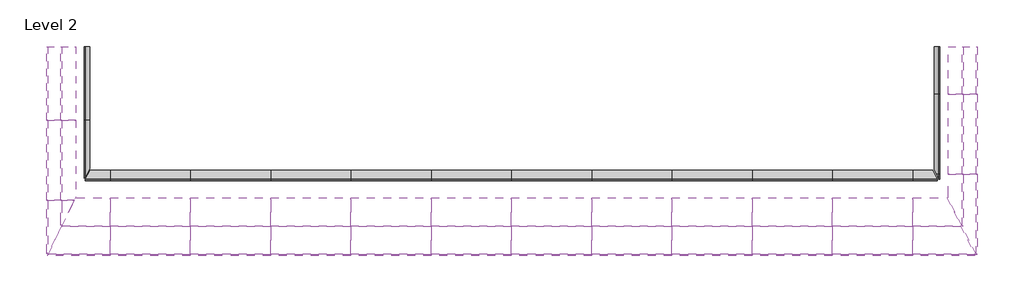
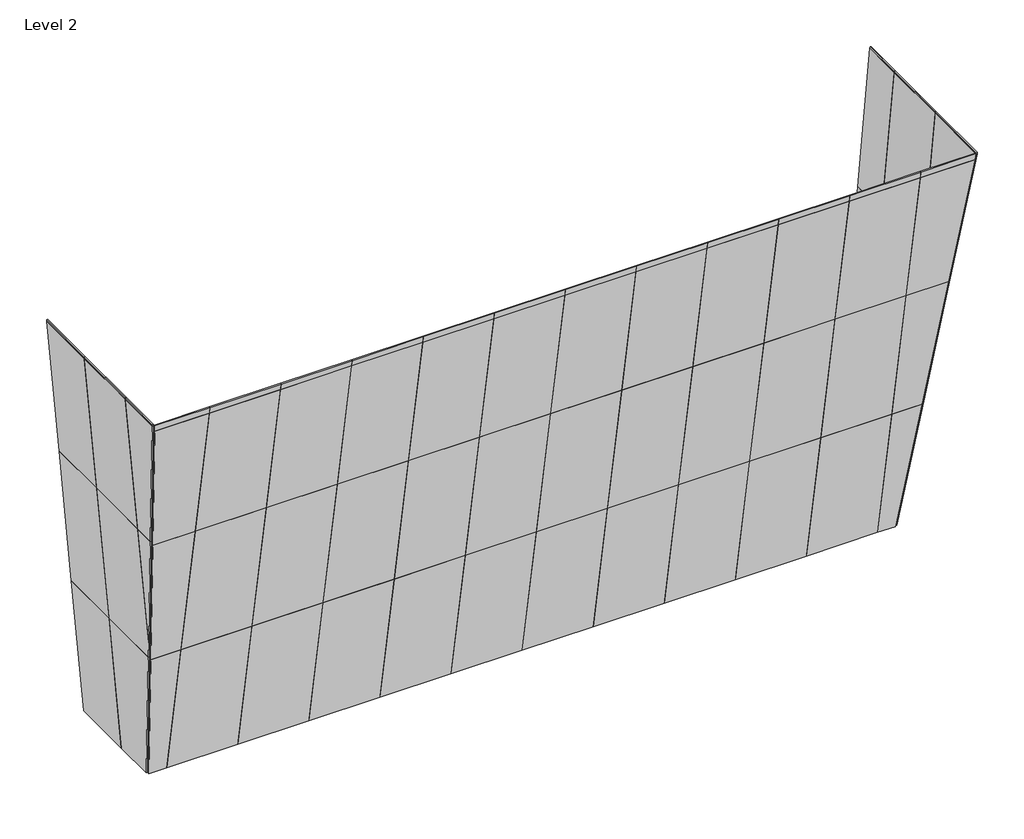
# One storey: 71 plates.
"""IFC4 building model written with IfcOpenShell, lengths in millimetres."""

import ifcopenshell
import ifcopenshell.guid

model = None  # the IFC model being written
_history = None  # IfcOwnerHistory: only IFC2X3 demands one
_inside = {}  # id of a spatial element -> (the spatial element, [elements in it])
_under = {}  # id of a project, library or spatial element -> (it, [spatial elements below it])
_declared = {}  # id of a project -> (the project, [libraries it declares])
_typed = {}  # id of a type object -> (the type object, [elements of that type])
_made_of = {}  # id of a material, layer set ... -> (it, [elements and type objects made of it])


def new_model(schema):
    """Start an empty IFC model of exactly this schema.

    Asked for "IFC4X3", IfcOpenShell would pick the latest addendum, in which some entities
    have other attributes; the version numbers below select the first issue.
    IFC2X3 requires an IfcOwnerHistory on every rooted entity: one is made here for all.
    """
    global model, _history
    if schema == "IFC4X3":
        model = ifcopenshell.file(schema_version=(4, 3, 0, 0))
    else:
        model = ifcopenshell.file(schema=schema)
    _inside.clear()
    _under.clear()
    _declared.clear()
    _typed.clear()
    _made_of.clear()
    _history = None
    if model.schema == "IFC2X3":
        org = make("IfcOrganization", Name="unknown")
        user = make(
            "IfcPersonAndOrganization",
            ThePerson=make("IfcPerson", FamilyName="unknown"),
            TheOrganization=org,
        )
        app = make(
            "IfcApplication",
            ApplicationDeveloper=org,
            Version="unknown",
            ApplicationFullName="unknown",
            ApplicationIdentifier="unknown",
        )
        _history = make(
            "IfcOwnerHistory",
            OwningUser=user,
            OwningApplication=app,
            ChangeAction="ADDED",
            CreationDate=0,
        )
    return model


def make(cls, **values):
    """One entity of the class cls with the attributes given. An attribute that is None is left unset."""
    return model.create_entity(
        cls, **{name: value for name, value in values.items() if value is not None}
    )


def rooted(cls, **values):
    """An entity with a GlobalId (a new one), such as an element, a storey or a relation."""
    return make(cls, GlobalId=ifcopenshell.guid.new(), OwnerHistory=_history, **values)


def si_unit(unit_type, name, prefix=None):
    """IfcSIUnit, for example si_unit("LENGTHUNIT", "METRE", prefix="MILLI")."""
    return make("IfcSIUnit", UnitType=unit_type, Prefix=prefix, Name=name)


def assignment(units):
    """IfcUnitAssignment: the units of a project."""
    return None if units is None else make("IfcUnitAssignment", Units=units)


def point(xyz):
    """IfcCartesianPoint."""
    return None if xyz is None else make("IfcCartesianPoint", Coordinates=xyz)


def direction(xyz):
    """IfcDirection."""
    return None if xyz is None else make("IfcDirection", DirectionRatios=xyz)


def frame(location, z_axis=None, x_axis=None):
    """IfcAxis2Placement3D, a coordinate frame: its origin and axes. An axis left out is left unset."""
    return make(
        "IfcAxis2Placement3D",
        Location=point(location),
        Axis=direction(z_axis),
        RefDirection=direction(x_axis),
    )


def origin():
    """The frame at (0, 0, 0) with its axes left unset."""
    return frame((0.0, 0.0, 0.0))


def origin_with_axes():
    """The frame at (0, 0, 0) with the z axis (0, 0, 1) and the x axis (1, 0, 0) written out."""
    return frame((0.0, 0.0, 0.0), z_axis=(0.0, 0.0, 1.0), x_axis=(1.0, 0.0, 0.0))


def place(relative_to, where):
    """IfcLocalPlacement: puts the frame where relative to a parent placement (None: the world)."""
    return make(
        "IfcLocalPlacement", PlacementRelTo=relative_to, RelativePlacement=where
    )


def context(
    kind, dimensions, precision=None, world=None, true_north=None, identifier=None
):
    """IfcGeometricRepresentationContext, for example the 3D "Model" context."""
    return make(
        "IfcGeometricRepresentationContext",
        ContextIdentifier=identifier,
        ContextType=kind,
        CoordinateSpaceDimension=dimensions,
        Precision=precision,
        WorldCoordinateSystem=world,
        TrueNorth=true_north,
    )


def project(units=None, contexts=None):
    """IfcProject with its units and contexts."""
    return rooted(
        "IfcProject",
        Name="project",
        RepresentationContexts=contexts,
        UnitsInContext=assignment(units),
    )


def spatial(cls, under=None, at=None, **own):
    """A site, building, storey or space (cls), placed at a placement, below another one or the project."""
    s = rooted(cls, ObjectPlacement=at, **own)
    if under is not None:
        _under.setdefault(under.id(), (under, []))[1].append(s)
    return s


def polyline(points):
    """IfcPolyline through the points."""
    return make("IfcPolyline", Points=[point(p) for p in points])


def outline(outer, holes=None, kind="AREA"):
    """IfcArbitraryClosedProfileDef: a profile drawn as a closed curve; with holes, ...WithVoids."""
    if holes is None:
        return make("IfcArbitraryClosedProfileDef", ProfileType=kind, OuterCurve=outer)
    return make(
        "IfcArbitraryProfileDefWithVoids",
        ProfileType=kind,
        OuterCurve=outer,
        InnerCurves=holes,
    )


def extrude(swept, where, along, depth):
    """IfcExtrudedAreaSolid: the profile swept, set in the frame where, extruded along a direction by depth."""
    return make(
        "IfcExtrudedAreaSolid",
        SweptArea=swept,
        Position=where,
        ExtrudedDirection=direction(along),
        Depth=depth,
    )


def shape(context_of_items, identifier, shape_type, items):
    """IfcShapeRepresentation: the items that make up one representation, for example the "Body"."""
    return make(
        "IfcShapeRepresentation",
        ContextOfItems=context_of_items,
        RepresentationIdentifier=identifier,
        RepresentationType=shape_type,
        Items=items,
    )


def source(mapping_origin, context_of_items, identifier, shape_type, items):
    """IfcRepresentationMap: a shape defined once, which mapped items show again and again."""
    return make(
        "IfcRepresentationMap",
        MappingOrigin=mapping_origin,
        MappedRepresentation=shape(context_of_items, identifier, shape_type, items),
    )


def transform(
    local_origin,
    x_axis=None,
    y_axis=None,
    z_axis=None,
    scale=None,
    scale2=None,
    scale3=None,
    uniform=True,
):
    """IfcCartesianTransformationOperator3D, or its non-uniform kind. x_axis, y_axis, z_axis: its Axis1, 2, 3."""
    if uniform:
        return make(
            "IfcCartesianTransformationOperator3D",
            Axis1=direction(x_axis),
            Axis2=direction(y_axis),
            LocalOrigin=point(local_origin),
            Scale=scale,
            Axis3=direction(z_axis),
        )
    return make(
        "IfcCartesianTransformationOperator3DnonUniform",
        Axis1=direction(x_axis),
        Axis2=direction(y_axis),
        LocalOrigin=point(local_origin),
        Scale=scale,
        Axis3=direction(z_axis),
        Scale2=scale2,
        Scale3=scale3,
    )


def mapped(mapping_source, mapping_target):
    """IfcMappedItem: shows the shape of a source again, moved by a transform."""
    return make(
        "IfcMappedItem", MappingSource=mapping_source, MappingTarget=mapping_target
    )


def made_of(thing, what):
    """Note that an element or type object is made of a material, layer set ...; save() writes the relation."""
    if what is not None:
        _made_of.setdefault(what.id(), (what, []))[1].append(thing)
    return thing


def element(
    cls,
    number,
    at=None,
    inside=None,
    cuts=None,
    type_object=None,
    material=None,
    context=None,
    identifier="Body",
    shape_type=None,
    held_by="IfcProductDefinitionShape",
    body=None,
    shapes=None,
    **own,
):
    """One element of the class cls, such as IfcWall. Its Tag is "e" and its number.

    at: its placement. inside: the storey or other place that contains it. cuts: it is an
    opening in that element (IfcRelVoidsElement). A single representation is given by context,
    identifier, shape_type and body (its items); several are given by shapes. held_by: the class
    of the entity that holds the representations. save() writes the other relations.
    """
    e = rooted(cls, Tag="e%d" % number, ObjectPlacement=at, **own)
    if body is not None:
        shapes = [shape(context, identifier, shape_type, body)]
    if shapes is not None:
        e.Representation = make(held_by, Representations=shapes)
    if inside is not None:
        _inside.setdefault(inside.id(), (inside, []))[1].append(e)
    if cuts is not None:
        rooted(
            "IfcRelVoidsElement", RelatingBuildingElement=cuts, RelatedOpeningElement=e
        )
    if type_object is not None:
        _typed.setdefault(type_object.id(), (type_object, []))[1].append(e)
    return made_of(e, material)


def aggregate(whole, parts):
    """IfcRelAggregates: a whole, such as a stair, and the parts it consists of."""
    return rooted("IfcRelAggregates", RelatingObject=whole, RelatedObjects=parts)


def save(model, path):
    """Write the relations noted so far, then the file.

    IfcRelAggregates (storeys below a building ...), IfcRelContainedInSpatialStructure (elements
    in a storey), IfcRelDefinesByType, IfcRelAssociatesMaterial and IfcRelDeclares: one each for
    every whole, place, type object, material and project.
    """
    for whole, parts in _under.values():
        aggregate(whole, parts)
    for where, things in _inside.values():
        rooted(
            "IfcRelContainedInSpatialStructure",
            RelatedElements=things,
            RelatingStructure=where,
        )
    for kind, things in _typed.values():
        rooted("IfcRelDefinesByType", RelatedObjects=things, RelatingType=kind)
    for what, things in _made_of.values():
        rooted("IfcRelAssociatesMaterial", RelatedObjects=things, RelatingMaterial=what)
    for by, libraries in _declared.values():
        rooted("IfcRelDeclares", RelatingContext=by, RelatedDefinitions=libraries)
    model.write(path)


def system_panel_glazed_2e91cb65(model_context):
    return source(origin(), model_context, "Body", "SweptSolid", [
        extrude(outline(polyline([(838.2000002, -44.45), (-838.2000002, -44.45), (-838.2000002, -19.05), (838.2000002, -19.05), (838.2000002, -44.45)])), origin_with_axes(), (0.0, 0.0, 1.0), 3657.6),
    ])


def system_panel_glazed_41c8569a(model_context):
    return source(origin(), model_context, "Body", "SweptSolid", [
        extrude(outline(polyline([(3054.1438606, -268.2393521), (0.0, 268.2393521), (3054.1438606, 268.2393521), (3054.1438606, -268.2393521)])), frame((0.0, -44.45, 0.0), z_axis=(0.0, 1.0, 0.0), x_axis=(0.0, 0.0, 1.0)), (0.0, 0.0, 1.0), 25.4),
    ])


def system_panel_glazed_1f34555f(model_context):
    return source(origin(), model_context, "Body", "SweptSolid", [
        extrude(outline(polyline([(914.4, -44.45), (-914.4, -44.45), (-914.4, -19.05), (914.4, -19.05), (914.4, -44.45)])), origin_with_axes(), (0.0, 0.0, 1.0), 3657.6),
    ])


def system_panel_glazed_8b4ddac8(model_context):
    return source(origin(), model_context, "Body", "SweptSolid", [
        extrude(outline(polyline([(838.2000002, -44.45), (-838.2000002, -44.45), (-838.2000002, -19.05), (838.2000002, -19.05), (838.2000002, -44.45)])), origin_with_axes(), (0.0, 0.0, 1.0), 41.9143134),
    ])


def system_panel_glazed_7f82afe2(model_context):
    return source(origin(), model_context, "Body", "SweptSolid", [
        extrude(outline(polyline([(914.4, -44.45), (-914.4, -44.45), (-914.4, -19.05), (914.4, -19.05), (914.4, -44.45)])), origin_with_axes(), (0.0, 0.0, 1.0), 41.9143134),
    ])


def system_panel_glazed_f4345ae3(model_context):
    return source(origin(), model_context, "Body", "SweptSolid", [
        extrude(outline(polyline([(914.4, -44.45), (-914.4, -44.45), (-914.4, -19.05), (914.4, -19.05), (914.4, -44.45)])), origin_with_axes(), (0.0, 0.0, 1.0), 169.2731269),
    ])


def system_panel_glazed_866ab655(model_context):
    return source(origin(), model_context, "Body", "SweptSolid", [
        extrude(outline(polyline([(0.0, -808.3993064), (0.0, 914.4), (3657.6, 914.4), (3657.6, -914.4), (603.4561394, -914.4), (0.0, -808.3993064)])), frame((0.0, -44.45, 0.0), z_axis=(0.0, 1.0, 0.0), x_axis=(0.0, 0.0, 1.0)), (0.0, 0.0, 1.0), 25.4),
    ])


def system_panel_glazed_bcd6892e(model_context):
    return source(origin(), model_context, "Body", "SweptSolid", [
        extrude(outline(polyline([(0.0, 53.0003468), (0.0, 589.4790509), (3657.6, 589.4790509), (3657.6, -589.4790509), (0.0, 53.0003468)])), frame((0.0, -44.45, 0.0), z_axis=(0.0, 1.0, 0.0), x_axis=(0.0, 0.0, 1.0)), (0.0, 0.0, 1.0), 25.4),
    ])


def system_panel_glazed_e7bd2299(model_context):
    return source(origin(), model_context, "Body", "SweptSolid", [
        extrude(outline(polyline([(0.0, -268.2393521), (0.0, 910.7187498), (3657.6, 910.7187498), (3657.6, -910.7187498), (0.0, -268.2393521)])), frame((0.0, -44.45, 0.0), z_axis=(0.0, 1.0, 0.0), x_axis=(0.0, 0.0, 1.0)), (0.0, 0.0, 1.0), 25.4),
    ])


def system_panel_glazed_0a43eb3e(model_context):
    return source(origin(), model_context, "Body", "SweptSolid", [
        extrude(outline(polyline([(0.0, -907.0374994), (0.0, 914.4000002), (41.9143134, 914.4000002), (41.9143134, -914.4000002), (0.0, -907.0374994)])), frame((0.0, -44.45, 0.0), z_axis=(0.0, 1.0, 0.0), x_axis=(0.0, 0.0, 1.0)), (0.0, 0.0, 1.0), 25.4),
    ])


def system_panel_glazed_35afb83b(model_context):
    return source(origin(), model_context, "Body", "SweptSolid", [
        extrude(outline(polyline([(0.0, -71.0314805), (0.0, 386.1685195), (3657.6, 386.1685195), (3657.6, -386.1685195), (0.0, -71.0314805)])), frame((0.0, -44.45, 0.0), z_axis=(0.0, 1.0, 0.0), x_axis=(0.0, 0.0, 1.0)), (0.0, 0.0, 1.0), 25.4),
    ])


def system_panel_glazed_ca25d662(model_context):
    return source(origin(), model_context, "Body", "SweptSolid", [
        extrude(outline(polyline([(0.0, -386.1685195), (0.0, 71.0314805), (3657.6, 386.1685195), (3657.6, -386.1685195), (0.0, -386.1685195)])), frame((0.0, -44.45, 0.0), z_axis=(0.0, 1.0, 0.0), x_axis=(0.0, 0.0, 1.0)), (0.0, 0.0, 1.0), 25.4),
    ])


def system_panel_glazed_d5b9b34d(model_context):
    return source(origin(), model_context, "Body", "SweptSolid", [
        extrude(outline(polyline([(0.0, -228.6), (0.0, 543.7370389), (3657.6, 543.7370389), (3657.6, -543.7370389), (0.0, -228.6)])), frame((0.0, -44.45, 0.0), z_axis=(0.0, 1.0, 0.0), x_axis=(0.0, 0.0, 1.0)), (0.0, 0.0, 1.0), 25.4),
    ])


def system_panel_glazed_127879aa(model_context):
    return source(origin(), model_context, "Body", "SweptSolid", [
        extrude(outline(polyline([(0.0, -543.7370389), (0.0, 228.6), (3657.6, 543.7370389), (3657.6, -543.7370389), (0.0, -543.7370389)])), frame((0.0, -44.45, 0.0), z_axis=(0.0, 1.0, 0.0), x_axis=(0.0, 0.0, 1.0)), (0.0, 0.0, 1.0), 25.4),
    ])


def system_panel_glazed_cde5e94a(model_context):
    return source(origin(), model_context, "Body", "SweptSolid", [
        extrude(outline(polyline([(0.0, -386.1685195), (0.0, 701.3055584), (3657.6, 701.3055584), (3657.6, -701.3055584), (0.0, -386.1685195)])), frame((0.0, -44.45, 0.0), z_axis=(0.0, 1.0, 0.0), x_axis=(0.0, 0.0, 1.0)), (0.0, 0.0, 1.0), 25.4),
    ])


def system_panel_glazed_b3fa7013(model_context):
    return source(origin(), model_context, "Body", "SweptSolid", [
        extrude(outline(polyline([(0.0, -701.3055584), (0.0, 386.1685195), (3657.6, 701.3055584), (3657.6, -701.3055584), (0.0, -701.3055584)])), frame((0.0, -44.45, 0.0), z_axis=(0.0, 1.0, 0.0), x_axis=(0.0, 0.0, 1.0)), (0.0, 0.0, 1.0), 25.4),
    ])


def system_panel_glazed_d86b06c2(model_context):
    return source(origin(), model_context, "Body", "SweptSolid", [
        extrude(outline(polyline([(0.0, -694.0133132), (0.0, 708.5978036), (169.2731269, 708.5978036), (169.2731269, -708.5978036), (0.0, -694.0133132)])), frame((0.0, -44.45, 0.0), z_axis=(0.0, 1.0, 0.0), x_axis=(0.0, 0.0, 1.0)), (0.0, 0.0, 1.0), 25.4),
    ])


def system_panel_glazed_9c30f1a4(model_context):
    return source(origin(), model_context, "Body", "SweptSolid", [
        extrude(outline(polyline([(0.0, -708.5978036), (0.0, 694.0133132), (169.2731269, 708.5978036), (169.2731269, -708.5978036), (0.0, -708.5978036)])), frame((0.0, -44.45, 0.0), z_axis=(0.0, 1.0, 0.0), x_axis=(0.0, 0.0, 1.0)), (0.0, 0.0, 1.0), 25.4),
    ])


def system_panel_glazed_d54edbd1(model_context):
    return source(origin(), model_context, "Body", "SweptSolid", [
        extrude(outline(polyline([(0.0, -873.5917397), (0.0, 231.112342), (3657.6, 873.5917397), (3657.6, -873.5917397), (0.0, -873.5917397)])), frame((0.0, -44.45, 0.0), z_axis=(0.0, 1.0, 0.0), x_axis=(0.0, 0.0, 1.0)), (0.0, 0.0, 1.0), 25.4),
    ])


def system_panel_glazed_959d3605(model_context):
    return source(origin(), model_context, "Body", "SweptSolid", [
        extrude(outline(polyline([(0.0, -914.4), (0.0, 832.7834794), (464.6383785, 914.4), (3657.6, 914.4), (3657.6, -914.4), (0.0, -914.4)])), frame((0.0, -44.45, 0.0), z_axis=(0.0, 1.0, 0.0), x_axis=(0.0, 0.0, 1.0)), (0.0, 0.0, 1.0), 25.4),
    ])


def system_panel_glazed_04b02cc8(model_context):
    return source(origin(), model_context, "Body", "SweptSolid", [
        extrude(outline(polyline([(0.0, -280.4314386), (3192.9616215, 280.4314386), (3192.9616215, -280.4314386), (0.0, -280.4314386)])), frame((0.0, -44.45, 0.0), z_axis=(0.0, 1.0, 0.0), x_axis=(0.0, 0.0, 1.0)), (0.0, 0.0, 1.0), 25.4),
    ])


def system_panel_glazed_cd333de7(model_context):
    return source(origin(), model_context, "Body", "SweptSolid", [
        extrude(outline(polyline([(0.0, -601.6711374), (0.0, -40.8082603), (3657.6, 601.6711374), (3657.6, -601.6711374), (0.0, -601.6711374)])), frame((0.0, -44.45, 0.0), z_axis=(0.0, 1.0, 0.0), x_axis=(0.0, 0.0, 1.0)), (0.0, 0.0, 1.0), 25.4),
    ])


def system_panel_glazed_abe217f1(model_context):
    return source(origin(), model_context, "Body", "SweptSolid", [
        extrude(outline(polyline([(0.0, -605.3523878), (0.0, 597.989887), (41.9143134, 605.3523878), (41.9143134, -605.3523878), (0.0, -605.3523878)])), frame((0.0, -44.45, 0.0), z_axis=(0.0, 1.0, 0.0), x_axis=(0.0, 0.0, 1.0)), (0.0, 0.0, 1.0), 25.4),
    ])


def system_panel_glazed_44e43824(model_context):
    return source(origin(), model_context, "Body", "SweptSolid", [
        extrude(outline(polyline([(542.0483058, -44.45), (-542.0483058, -44.45), (-542.0483058, -19.05), (542.0483058, -19.05), (542.0483058, -44.45)])), origin_with_axes(), (0.0, 0.0, 1.0), 3657.6),
    ])


def system_panel_glazed_5c475300(model_context):
    return source(origin(), model_context, "Body", "SweptSolid", [
        extrude(outline(polyline([(542.0483058, -44.45), (-542.0483058, -44.45), (-542.0483058, -19.05), (542.0483058, -19.05), (542.0483058, -44.45)])), origin_with_axes(), (0.0, 0.0, 1.0), 41.9143134),
    ])


model = new_model("IFC4")

# Units and contexts
model_context = context("Model", 3, world=origin())
ifc_project = project(units=[si_unit("LENGTHUNIT", "METRE", prefix="MILLI")], contexts=[model_context])

# Site, building, storey
site = spatial("IfcSite", under=ifc_project)
building = spatial("IfcBuilding", under=site)
storey = spatial("IfcBuildingStorey", under=building, Name="Level 2", Elevation=3657.6)

# Plates
placement = place(None, origin())
system_panel_glazed_shape = system_panel_glazed_2e91cb65(model_context)
element("IfcPlate", 1, ObjectType="System Panel : Glazed", at=placement, inside=storey, context=model_context, shape_type="MappedRepresentation", body=[
    mapped(system_panel_glazed_shape, transform((-10766.9154339, -10596.6984697, 3656.4931221), x_axis=(0.0, -1.0, 0.0), y_axis=(0.9961946980917455, 0.0, 0.08715574274765803), z_axis=(-0.08715574274765803, 0.0, 0.9961946980917455))),
])
element("IfcPlate", 2, ObjectType="System Panel : Glazed", at=placement, inside=storey, context=model_context, shape_type="MappedRepresentation", body=[
    mapped(system_panel_glazed_shape, transform((-11085.6962786, -10596.6984697, 7300.1748498), x_axis=(0.0, -1.0, 0.0), y_axis=(0.9961946980917455, 0.0, 0.08715574274765803), z_axis=(-0.08715574274765803, 0.0, 0.9961946980917455))),
])
element("IfcPlate", 3, ObjectType="System Panel : Glazed", at=placement, inside=storey, context=model_context, shape_type="MappedRepresentation", body=[
    mapped(system_panel_glazed_shape, transform((-11404.4771233, -10596.6984697, 10943.8565775), x_axis=(0.0, -1.0, 0.0), y_axis=(0.9961946980917455, 0.0, 0.08715574274765803), z_axis=(-0.08715574274765803, 0.0, 0.9961946980917455))),
])
system_panel_glazed_2_shape = system_panel_glazed_41c8569a(model_context)
element("IfcPlate", 4, ObjectType="System Panel : Glazed", at=placement, inside=storey, context=model_context, shape_type="MappedRepresentation", body=[
    mapped(system_panel_glazed_2_shape, transform((8487.8855556, -12939.6344332, 4257.6529286), x_axis=(0.0, 1.0, 0.0), y_axis=(-0.9961946980917455, 0.0, 0.08715574274765803), z_axis=(0.08715574274765803, 0.0, 0.9961946980917455))),
])
system_panel_glazed_3_shape = system_panel_glazed_1f34555f(model_context)
element("IfcPlate", 5, ObjectType="System Panel : Glazed", at=placement, inside=storey, context=model_context, shape_type="MappedRepresentation", body=[
    mapped(system_panel_glazed_3_shape, transform((-11404.4771233, -12349.2984699, 10943.8565775), x_axis=(0.0, -1.0, 0.0), y_axis=(0.9961946980917455, 0.0, 0.08715574274765803), z_axis=(-0.08715574274765803, 0.0, 0.9961946980917455))),
])
element("IfcPlate", 6, ObjectType="System Panel : Glazed", at=placement, inside=storey, context=model_context, shape_type="MappedRepresentation", body=[
    mapped(system_panel_glazed_3_shape, transform((-9408.1607851, -12552.1096101, 3655.3946681), x_axis=(1.0, 0.0, 0.0), y_axis=(0.0, 0.9848077530122081, 0.17364817766693014), z_axis=(0.0, -0.17364817766693014, 0.9848077530122081))),
])
element("IfcPlate", 7, ObjectType="System Panel : Glazed", at=placement, inside=storey, context=model_context, shape_type="MappedRepresentation", body=[
    mapped(system_panel_glazed_3_shape, transform((-7579.3607851, -12552.1096101, 3655.3946681), x_axis=(1.0, 0.0, 0.0), y_axis=(0.0, 0.9848077530122081, 0.17364817766693014), z_axis=(0.0, -0.17364817766693014, 0.9848077530122081))),
])
element("IfcPlate", 8, ObjectType="System Panel : Glazed", at=placement, inside=storey, context=model_context, shape_type="MappedRepresentation", body=[
    mapped(system_panel_glazed_3_shape, transform((-5750.5607851, -12552.1096101, 3655.3946681), x_axis=(1.0, 0.0, 0.0), y_axis=(0.0, 0.9848077530122081, 0.17364817766693014), z_axis=(0.0, -0.17364817766693014, 0.9848077530122081))),
])
element("IfcPlate", 9, ObjectType="System Panel : Glazed", at=placement, inside=storey, context=model_context, shape_type="MappedRepresentation", body=[
    mapped(system_panel_glazed_3_shape, transform((-3921.7607851, -12552.1096101, 3655.3946681), x_axis=(1.0, 0.0, 0.0), y_axis=(0.0, 0.9848077530122081, 0.17364817766693014), z_axis=(0.0, -0.17364817766693014, 0.9848077530122081))),
])
element("IfcPlate", 10, ObjectType="System Panel : Glazed", at=placement, inside=storey, context=model_context, shape_type="MappedRepresentation", body=[
    mapped(system_panel_glazed_3_shape, transform((-2092.9607851, -12552.1096101, 3655.3946681), x_axis=(1.0, 0.0, 0.0), y_axis=(0.0, 0.9848077530122081, 0.17364817766693014), z_axis=(0.0, -0.17364817766693014, 0.9848077530122081))),
])
element("IfcPlate", 11, ObjectType="System Panel : Glazed", at=placement, inside=storey, context=model_context, shape_type="MappedRepresentation", body=[
    mapped(system_panel_glazed_3_shape, transform((-264.1607851, -12552.1096101, 3655.3946681), x_axis=(1.0, 0.0, 0.0), y_axis=(0.0, 0.9848077530122081, 0.17364817766693014), z_axis=(0.0, -0.17364817766693014, 0.9848077530122081))),
])
element("IfcPlate", 12, ObjectType="System Panel : Glazed", at=placement, inside=storey, context=model_context, shape_type="MappedRepresentation", body=[
    mapped(system_panel_glazed_3_shape, transform((1564.6392149, -12552.1096101, 3655.3946681), x_axis=(1.0, 0.0, 0.0), y_axis=(0.0, 0.9848077530122081, 0.17364817766693014), z_axis=(0.0, -0.17364817766693014, 0.9848077530122081))),
])
element("IfcPlate", 13, ObjectType="System Panel : Glazed", at=placement, inside=storey, context=model_context, shape_type="MappedRepresentation", body=[
    mapped(system_panel_glazed_3_shape, transform((3393.4392149, -12552.1096101, 3655.3946681), x_axis=(1.0, 0.0, 0.0), y_axis=(0.0, 0.9848077530122081, 0.17364817766693014), z_axis=(0.0, -0.17364817766693014, 0.9848077530122081))),
])
element("IfcPlate", 14, ObjectType="System Panel : Glazed", at=placement, inside=storey, context=model_context, shape_type="MappedRepresentation", body=[
    mapped(system_panel_glazed_3_shape, transform((5222.2392149, -12552.1096101, 3655.3946681), x_axis=(1.0, 0.0, 0.0), y_axis=(0.0, 0.9848077530122081, 0.17364817766693014), z_axis=(0.0, -0.17364817766693014, 0.9848077530122081))),
])
element("IfcPlate", 15, ObjectType="System Panel : Glazed", at=placement, inside=storey, context=model_context, shape_type="MappedRepresentation", body=[
    mapped(system_panel_glazed_3_shape, transform((7051.0392149, -12552.1096101, 3655.3946681), x_axis=(1.0, 0.0, 0.0), y_axis=(0.0, 0.9848077530122081, 0.17364817766693014), z_axis=(0.0, -0.17364817766693014, 0.9848077530122081))),
])
element("IfcPlate", 16, ObjectType="System Panel : Glazed", at=placement, inside=storey, context=model_context, shape_type="MappedRepresentation", body=[
    mapped(system_panel_glazed_3_shape, transform((-9408.1607851, -13187.2451847, 7257.4275056), x_axis=(1.0, 0.0, 0.0), y_axis=(0.0, 0.9848077530122081, 0.17364817766693014), z_axis=(0.0, -0.17364817766693014, 0.9848077530122081))),
])
element("IfcPlate", 17, ObjectType="System Panel : Glazed", at=placement, inside=storey, context=model_context, shape_type="MappedRepresentation", body=[
    mapped(system_panel_glazed_3_shape, transform((-7579.3607851, -13187.2451847, 7257.4275056), x_axis=(1.0, 0.0, 0.0), y_axis=(0.0, 0.9848077530122081, 0.17364817766693014), z_axis=(0.0, -0.17364817766693014, 0.9848077530122081))),
])
element("IfcPlate", 18, ObjectType="System Panel : Glazed", at=placement, inside=storey, context=model_context, shape_type="MappedRepresentation", body=[
    mapped(system_panel_glazed_3_shape, transform((-5750.5607851, -13187.2451847, 7257.4275056), x_axis=(1.0, 0.0, 0.0), y_axis=(0.0, 0.9848077530122081, 0.17364817766693014), z_axis=(0.0, -0.17364817766693014, 0.9848077530122081))),
])
element("IfcPlate", 19, ObjectType="System Panel : Glazed", at=placement, inside=storey, context=model_context, shape_type="MappedRepresentation", body=[
    mapped(system_panel_glazed_3_shape, transform((-3921.7607851, -13187.2451847, 7257.4275056), x_axis=(1.0, 0.0, 0.0), y_axis=(0.0, 0.9848077530122081, 0.17364817766693014), z_axis=(0.0, -0.17364817766693014, 0.9848077530122081))),
])
element("IfcPlate", 20, ObjectType="System Panel : Glazed", at=placement, inside=storey, context=model_context, shape_type="MappedRepresentation", body=[
    mapped(system_panel_glazed_3_shape, transform((-2092.9607851, -13187.2451847, 7257.4275056), x_axis=(1.0, 0.0, 0.0), y_axis=(0.0, 0.9848077530122081, 0.17364817766693014), z_axis=(0.0, -0.17364817766693014, 0.9848077530122081))),
])
element("IfcPlate", 21, ObjectType="System Panel : Glazed", at=placement, inside=storey, context=model_context, shape_type="MappedRepresentation", body=[
    mapped(system_panel_glazed_3_shape, transform((-264.1607851, -13187.2451847, 7257.4275056), x_axis=(1.0, 0.0, 0.0), y_axis=(0.0, 0.9848077530122081, 0.17364817766693014), z_axis=(0.0, -0.17364817766693014, 0.9848077530122081))),
])
element("IfcPlate", 22, ObjectType="System Panel : Glazed", at=placement, inside=storey, context=model_context, shape_type="MappedRepresentation", body=[
    mapped(system_panel_glazed_3_shape, transform((1564.6392149, -13187.2451847, 7257.4275056), x_axis=(1.0, 0.0, 0.0), y_axis=(0.0, 0.9848077530122081, 0.17364817766693014), z_axis=(0.0, -0.17364817766693014, 0.9848077530122081))),
])
element("IfcPlate", 23, ObjectType="System Panel : Glazed", at=placement, inside=storey, context=model_context, shape_type="MappedRepresentation", body=[
    mapped(system_panel_glazed_3_shape, transform((3393.4392149, -13187.2451847, 7257.4275056), x_axis=(1.0, 0.0, 0.0), y_axis=(0.0, 0.9848077530122081, 0.17364817766693014), z_axis=(0.0, -0.17364817766693014, 0.9848077530122081))),
])
element("IfcPlate", 24, ObjectType="System Panel : Glazed", at=placement, inside=storey, context=model_context, shape_type="MappedRepresentation", body=[
    mapped(system_panel_glazed_3_shape, transform((5222.2392149, -13187.2451847, 7257.4275056), x_axis=(1.0, 0.0, 0.0), y_axis=(0.0, 0.9848077530122081, 0.17364817766693014), z_axis=(0.0, -0.17364817766693014, 0.9848077530122081))),
])
element("IfcPlate", 25, ObjectType="System Panel : Glazed", at=placement, inside=storey, context=model_context, shape_type="MappedRepresentation", body=[
    mapped(system_panel_glazed_3_shape, transform((7051.0392149, -13187.2451847, 7257.4275056), x_axis=(1.0, 0.0, 0.0), y_axis=(0.0, 0.9848077530122081, 0.17364817766693014), z_axis=(0.0, -0.17364817766693014, 0.9848077530122081))),
])
element("IfcPlate", 26, ObjectType="System Panel : Glazed", at=placement, inside=storey, context=model_context, shape_type="MappedRepresentation", body=[
    mapped(system_panel_glazed_3_shape, transform((-9408.1607851, -13822.3807593, 10859.460343), x_axis=(1.0, 0.0, 0.0), y_axis=(0.0, 0.9848077530122081, 0.17364817766693014), z_axis=(0.0, -0.17364817766693014, 0.9848077530122081))),
])
element("IfcPlate", 27, ObjectType="System Panel : Glazed", at=placement, inside=storey, context=model_context, shape_type="MappedRepresentation", body=[
    mapped(system_panel_glazed_3_shape, transform((-7579.3607851, -13822.3807593, 10859.460343), x_axis=(1.0, 0.0, 0.0), y_axis=(0.0, 0.9848077530122081, 0.17364817766693014), z_axis=(0.0, -0.17364817766693014, 0.9848077530122081))),
])
element("IfcPlate", 28, ObjectType="System Panel : Glazed", at=placement, inside=storey, context=model_context, shape_type="MappedRepresentation", body=[
    mapped(system_panel_glazed_3_shape, transform((-5750.5607851, -13822.3807593, 10859.460343), x_axis=(1.0, 0.0, 0.0), y_axis=(0.0, 0.9848077530122081, 0.17364817766693014), z_axis=(0.0, -0.17364817766693014, 0.9848077530122081))),
])
element("IfcPlate", 29, ObjectType="System Panel : Glazed", at=placement, inside=storey, context=model_context, shape_type="MappedRepresentation", body=[
    mapped(system_panel_glazed_3_shape, transform((-3921.7607851, -13822.3807593, 10859.460343), x_axis=(1.0, 0.0, 0.0), y_axis=(0.0, 0.9848077530122081, 0.17364817766693014), z_axis=(0.0, -0.17364817766693014, 0.9848077530122081))),
])
element("IfcPlate", 30, ObjectType="System Panel : Glazed", at=placement, inside=storey, context=model_context, shape_type="MappedRepresentation", body=[
    mapped(system_panel_glazed_3_shape, transform((-2092.9607851, -13822.3807593, 10859.460343), x_axis=(1.0, 0.0, 0.0), y_axis=(0.0, 0.9848077530122081, 0.17364817766693014), z_axis=(0.0, -0.17364817766693014, 0.9848077530122081))),
])
element("IfcPlate", 31, ObjectType="System Panel : Glazed", at=placement, inside=storey, context=model_context, shape_type="MappedRepresentation", body=[
    mapped(system_panel_glazed_3_shape, transform((-264.1607851, -13822.3807593, 10859.460343), x_axis=(1.0, 0.0, 0.0), y_axis=(0.0, 0.9848077530122081, 0.17364817766693014), z_axis=(0.0, -0.17364817766693014, 0.9848077530122081))),
])
element("IfcPlate", 32, ObjectType="System Panel : Glazed", at=placement, inside=storey, context=model_context, shape_type="MappedRepresentation", body=[
    mapped(system_panel_glazed_3_shape, transform((1564.6392149, -13822.3807593, 10859.460343), x_axis=(1.0, 0.0, 0.0), y_axis=(0.0, 0.9848077530122081, 0.17364817766693014), z_axis=(0.0, -0.17364817766693014, 0.9848077530122081))),
])
element("IfcPlate", 33, ObjectType="System Panel : Glazed", at=placement, inside=storey, context=model_context, shape_type="MappedRepresentation", body=[
    mapped(system_panel_glazed_3_shape, transform((3393.4392149, -13822.3807593, 10859.460343), x_axis=(1.0, 0.0, 0.0), y_axis=(0.0, 0.9848077530122081, 0.17364817766693014), z_axis=(0.0, -0.17364817766693014, 0.9848077530122081))),
])
element("IfcPlate", 34, ObjectType="System Panel : Glazed", at=placement, inside=storey, context=model_context, shape_type="MappedRepresentation", body=[
    mapped(system_panel_glazed_3_shape, transform((5222.2392149, -13822.3807593, 10859.460343), x_axis=(1.0, 0.0, 0.0), y_axis=(0.0, 0.9848077530122081, 0.17364817766693014), z_axis=(0.0, -0.17364817766693014, 0.9848077530122081))),
])
element("IfcPlate", 35, ObjectType="System Panel : Glazed", at=placement, inside=storey, context=model_context, shape_type="MappedRepresentation", body=[
    mapped(system_panel_glazed_3_shape, transform((7051.0392149, -13822.3807593, 10859.460343), x_axis=(1.0, 0.0, 0.0), y_axis=(0.0, 0.9848077530122081, 0.17364817766693014), z_axis=(0.0, -0.17364817766693014, 0.9848077530122081))),
])
element("IfcPlate", 36, ObjectType="System Panel : Glazed", at=placement, inside=storey, context=model_context, shape_type="MappedRepresentation", body=[
    mapped(system_panel_glazed_3_shape, transform((8754.0717322, -11756.9950812, 7300.1748498), x_axis=(0.0, 1.0, 0.0), y_axis=(-0.9961946980917455, 0.0, 0.08715574274765803), z_axis=(0.08715574274765803, 0.0, 0.9961946980917455))),
])
element("IfcPlate", 37, ObjectType="System Panel : Glazed", at=placement, inside=storey, context=model_context, shape_type="MappedRepresentation", body=[
    mapped(system_panel_glazed_3_shape, transform((9072.8525769, -11756.9950812, 10943.8565775), x_axis=(0.0, 1.0, 0.0), y_axis=(-0.9961946980917455, 0.0, 0.08715574274765803), z_axis=(0.08715574274765803, 0.0, 0.9961946980917455))),
])
system_panel_glazed_4_shape = system_panel_glazed_8b4ddac8(model_context)
element("IfcPlate", 38, ObjectType="System Panel : Glazed", at=placement, inside=storey, context=model_context, shape_type="MappedRepresentation", body=[
    mapped(system_panel_glazed_4_shape, transform((-11723.2579679, -10596.6984697, 14587.5383053), x_axis=(0.0, -1.0, 0.0), y_axis=(0.9961946980917455, 0.0, 0.08715574274765803), z_axis=(-0.08715574274765803, 0.0, 0.9961946980917455))),
])
system_panel_glazed_5_shape = system_panel_glazed_7f82afe2(model_context)
element("IfcPlate", 39, ObjectType="System Panel : Glazed", at=placement, inside=storey, context=model_context, shape_type="MappedRepresentation", body=[
    mapped(system_panel_glazed_5_shape, transform((-11723.2579679, -12349.2984699, 14587.5383053), x_axis=(0.0, -1.0, 0.0), y_axis=(0.9961946980917455, 0.0, 0.08715574274765803), z_axis=(-0.08715574274765803, 0.0, 0.9961946980917455))),
])
element("IfcPlate", 40, ObjectType="System Panel : Glazed", at=placement, inside=storey, context=model_context, shape_type="MappedRepresentation", body=[
    mapped(system_panel_glazed_5_shape, transform((9391.6334216, -11756.9950812, 14587.5383053), x_axis=(0.0, 1.0, 0.0), y_axis=(-0.9961946980917455, 0.0, 0.08715574274765803), z_axis=(0.08715574274765803, 0.0, 0.9961946980917455))),
])
system_panel_glazed_6_shape = system_panel_glazed_f4345ae3(model_context)
element("IfcPlate", 41, ObjectType="System Panel : Glazed", at=placement, inside=storey, context=model_context, shape_type="MappedRepresentation", body=[
    mapped(system_panel_glazed_6_shape, transform((-9408.1607851, -14457.516334, 14461.4931804), x_axis=(1.0, 0.0, 0.0), y_axis=(0.0, 0.9848077530122081, 0.17364817766693014), z_axis=(0.0, -0.17364817766693014, 0.9848077530122081))),
])
element("IfcPlate", 42, ObjectType="System Panel : Glazed", at=placement, inside=storey, context=model_context, shape_type="MappedRepresentation", body=[
    mapped(system_panel_glazed_6_shape, transform((-7579.3607851, -14457.516334, 14461.4931804), x_axis=(1.0, 0.0, 0.0), y_axis=(0.0, 0.9848077530122081, 0.17364817766693014), z_axis=(0.0, -0.17364817766693014, 0.9848077530122081))),
])
element("IfcPlate", 43, ObjectType="System Panel : Glazed", at=placement, inside=storey, context=model_context, shape_type="MappedRepresentation", body=[
    mapped(system_panel_glazed_6_shape, transform((-5750.5607851, -14457.516334, 14461.4931804), x_axis=(1.0, 0.0, 0.0), y_axis=(0.0, 0.9848077530122081, 0.17364817766693014), z_axis=(0.0, -0.17364817766693014, 0.9848077530122081))),
])
element("IfcPlate", 44, ObjectType="System Panel : Glazed", at=placement, inside=storey, context=model_context, shape_type="MappedRepresentation", body=[
    mapped(system_panel_glazed_6_shape, transform((-3921.7607851, -14457.516334, 14461.4931804), x_axis=(1.0, 0.0, 0.0), y_axis=(0.0, 0.9848077530122081, 0.17364817766693014), z_axis=(0.0, -0.17364817766693014, 0.9848077530122081))),
])
element("IfcPlate", 45, ObjectType="System Panel : Glazed", at=placement, inside=storey, context=model_context, shape_type="MappedRepresentation", body=[
    mapped(system_panel_glazed_6_shape, transform((-2092.9607851, -14457.516334, 14461.4931804), x_axis=(1.0, 0.0, 0.0), y_axis=(0.0, 0.9848077530122081, 0.17364817766693014), z_axis=(0.0, -0.17364817766693014, 0.9848077530122081))),
])
element("IfcPlate", 46, ObjectType="System Panel : Glazed", at=placement, inside=storey, context=model_context, shape_type="MappedRepresentation", body=[
    mapped(system_panel_glazed_6_shape, transform((-264.1607851, -14457.516334, 14461.4931804), x_axis=(1.0, 0.0, 0.0), y_axis=(0.0, 0.9848077530122081, 0.17364817766693014), z_axis=(0.0, -0.17364817766693014, 0.9848077530122081))),
])
element("IfcPlate", 47, ObjectType="System Panel : Glazed", at=placement, inside=storey, context=model_context, shape_type="MappedRepresentation", body=[
    mapped(system_panel_glazed_6_shape, transform((1564.6392149, -14457.516334, 14461.4931804), x_axis=(1.0, 0.0, 0.0), y_axis=(0.0, 0.9848077530122081, 0.17364817766693014), z_axis=(0.0, -0.17364817766693014, 0.9848077530122081))),
])
element("IfcPlate", 48, ObjectType="System Panel : Glazed", at=placement, inside=storey, context=model_context, shape_type="MappedRepresentation", body=[
    mapped(system_panel_glazed_6_shape, transform((3393.4392149, -14457.516334, 14461.4931804), x_axis=(1.0, 0.0, 0.0), y_axis=(0.0, 0.9848077530122081, 0.17364817766693014), z_axis=(0.0, -0.17364817766693014, 0.9848077530122081))),
])
element("IfcPlate", 49, ObjectType="System Panel : Glazed", at=placement, inside=storey, context=model_context, shape_type="MappedRepresentation", body=[
    mapped(system_panel_glazed_6_shape, transform((5222.2392149, -14457.516334, 14461.4931804), x_axis=(1.0, 0.0, 0.0), y_axis=(0.0, 0.9848077530122081, 0.17364817766693014), z_axis=(0.0, -0.17364817766693014, 0.9848077530122081))),
])
element("IfcPlate", 50, ObjectType="System Panel : Glazed", at=placement, inside=storey, context=model_context, shape_type="MappedRepresentation", body=[
    mapped(system_panel_glazed_6_shape, transform((7051.0392149, -14457.516334, 14461.4931804), x_axis=(1.0, 0.0, 0.0), y_axis=(0.0, 0.9848077530122081, 0.17364817766693014), z_axis=(0.0, -0.17364817766693014, 0.9848077530122081))),
])
system_panel_glazed_7_shape = system_panel_glazed_866ab655(model_context)
element("IfcPlate", 51, ObjectType="System Panel : Glazed", at=placement, inside=storey, context=model_context, shape_type="MappedRepresentation", body=[
    mapped(system_panel_glazed_7_shape, transform((8435.2908875, -11756.9950812, 3656.4931221), x_axis=(0.0, 1.0, 0.0), y_axis=(-0.9961946980917455, 0.0, 0.08715574274765803), z_axis=(0.08715574274765803, 0.0, 0.9961946980917455))),
])
system_panel_glazed_8_shape = system_panel_glazed_bcd6892e(model_context)
element("IfcPlate", 52, ObjectType="System Panel : Glazed", at=placement, inside=storey, context=model_context, shape_type="MappedRepresentation", body=[
    mapped(system_panel_glazed_8_shape, transform((8754.0717322, -13260.8741321, 7300.1748498), x_axis=(0.0, 1.0, 0.0), y_axis=(-0.9961946980917455, 0.0, 0.08715574274765803), z_axis=(0.08715574274765803, 0.0, 0.9961946980917455))),
])
system_panel_glazed_9_shape = system_panel_glazed_e7bd2299(model_context)
element("IfcPlate", 53, ObjectType="System Panel : Glazed", at=placement, inside=storey, context=model_context, shape_type="MappedRepresentation", body=[
    mapped(system_panel_glazed_9_shape, transform((9072.8525769, -13582.1138309, 10943.8565775), x_axis=(0.0, 1.0, 0.0), y_axis=(-0.9961946980917455, 0.0, 0.08715574274765803), z_axis=(0.08715574274765803, 0.0, 0.9961946980917455))),
])
system_panel_glazed_10_shape = system_panel_glazed_0a43eb3e(model_context)
element("IfcPlate", 54, ObjectType="System Panel : Glazed", at=placement, inside=storey, context=model_context, shape_type="MappedRepresentation", body=[
    mapped(system_panel_glazed_10_shape, transform((9391.6334216, -13585.7950813, 14587.5383053), x_axis=(0.0, 1.0, 0.0), y_axis=(-0.9961946980917455, 0.0, 0.08715574274765803), z_axis=(0.08715574274765803, 0.0, 0.9961946980917455))),
])
system_panel_glazed_11_shape = system_panel_glazed_35afb83b(model_context)
element("IfcPlate", 55, ObjectType="System Panel : Glazed", at=placement, inside=storey, context=model_context, shape_type="MappedRepresentation", body=[
    mapped(system_panel_glazed_11_shape, transform((-10708.7293046, -12552.1096101, 3655.3946681), x_axis=(1.0, 0.0, 0.0), y_axis=(0.0, 0.9848077530122081, 0.17364817766693014), z_axis=(0.0, -0.17364817766693014, 0.9848077530122081))),
])
system_panel_glazed_12_shape = system_panel_glazed_ca25d662(model_context)
element("IfcPlate", 56, ObjectType="System Panel : Glazed", at=placement, inside=storey, context=model_context, shape_type="MappedRepresentation", body=[
    mapped(system_panel_glazed_12_shape, transform((8351.6077343, -12552.1096101, 3655.3946681), x_axis=(1.0, 0.0, 0.0), y_axis=(0.0, 0.9848077530122081, 0.17364817766693014), z_axis=(0.0, -0.17364817766693014, 0.9848077530122081))),
])
system_panel_glazed_13_shape = system_panel_glazed_d5b9b34d(model_context)
element("IfcPlate", 57, ObjectType="System Panel : Glazed", at=placement, inside=storey, context=model_context, shape_type="MappedRepresentation", body=[
    mapped(system_panel_glazed_13_shape, transform((-10866.2978241, -13187.2451847, 7257.4275056), x_axis=(1.0, 0.0, 0.0), y_axis=(0.0, 0.9848077530122081, 0.17364817766693014), z_axis=(0.0, -0.17364817766693014, 0.9848077530122081))),
])
system_panel_glazed_14_shape = system_panel_glazed_127879aa(model_context)
element("IfcPlate", 58, ObjectType="System Panel : Glazed", at=placement, inside=storey, context=model_context, shape_type="MappedRepresentation", body=[
    mapped(system_panel_glazed_14_shape, transform((8509.1762538, -13187.2451847, 7257.4275056), x_axis=(1.0, 0.0, 0.0), y_axis=(0.0, 0.9848077530122081, 0.17364817766693014), z_axis=(0.0, -0.17364817766693014, 0.9848077530122081))),
])
system_panel_glazed_15_shape = system_panel_glazed_cde5e94a(model_context)
element("IfcPlate", 59, ObjectType="System Panel : Glazed", at=placement, inside=storey, context=model_context, shape_type="MappedRepresentation", body=[
    mapped(system_panel_glazed_15_shape, transform((-11023.8663435, -13822.3807593, 10859.460343), x_axis=(1.0, 0.0, 0.0), y_axis=(0.0, 0.9848077530122081, 0.17364817766693014), z_axis=(0.0, -0.17364817766693014, 0.9848077530122081))),
])
system_panel_glazed_16_shape = system_panel_glazed_b3fa7013(model_context)
element("IfcPlate", 60, ObjectType="System Panel : Glazed", at=placement, inside=storey, context=model_context, shape_type="MappedRepresentation", body=[
    mapped(system_panel_glazed_16_shape, transform((8666.7447733, -13822.3807593, 10859.460343), x_axis=(1.0, 0.0, 0.0), y_axis=(0.0, 0.9848077530122081, 0.17364817766693014), z_axis=(0.0, -0.17364817766693014, 0.9848077530122081))),
])
system_panel_glazed_17_shape = system_panel_glazed_d86b06c2(model_context)
element("IfcPlate", 61, ObjectType="System Panel : Glazed", at=placement, inside=storey, context=model_context, shape_type="MappedRepresentation", body=[
    mapped(system_panel_glazed_17_shape, transform((-11031.1585887, -14457.516334, 14461.4931804), x_axis=(1.0, 0.0, 0.0), y_axis=(0.0, 0.9848077530122081, 0.17364817766693014), z_axis=(0.0, -0.17364817766693014, 0.9848077530122081))),
])
system_panel_glazed_18_shape = system_panel_glazed_9c30f1a4(model_context)
element("IfcPlate", 62, ObjectType="System Panel : Glazed", at=placement, inside=storey, context=model_context, shape_type="MappedRepresentation", body=[
    mapped(system_panel_glazed_18_shape, transform((8674.0370184, -14457.516334, 14461.4931804), x_axis=(1.0, 0.0, 0.0), y_axis=(0.0, 0.9848077530122081, 0.17364817766693014), z_axis=(0.0, -0.17364817766693014, 0.9848077530122081))),
])
system_panel_glazed_19_shape = system_panel_glazed_d54edbd1(model_context)
element("IfcPlate", 63, ObjectType="System Panel : Glazed", at=placement, inside=storey, context=model_context, shape_type="MappedRepresentation", body=[
    mapped(system_panel_glazed_19_shape, transform((-10766.9154339, -12308.4902096, 3656.4931221), x_axis=(0.0, -1.0, 0.0), y_axis=(0.9961946980917455, 0.0, 0.08715574274765803), z_axis=(-0.08715574274765803, 0.0, 0.9961946980917455))),
])
system_panel_glazed_20_shape = system_panel_glazed_959d3605(model_context)
element("IfcPlate", 64, ObjectType="System Panel : Glazed", at=placement, inside=storey, context=model_context, shape_type="MappedRepresentation", body=[
    mapped(system_panel_glazed_20_shape, transform((-11085.6962786, -12349.2984699, 7300.1748498), x_axis=(0.0, -1.0, 0.0), y_axis=(0.9961946980917455, 0.0, 0.08715574274765803), z_axis=(-0.08715574274765803, 0.0, 0.9961946980917455))),
])
system_panel_glazed_21_shape = system_panel_glazed_04b02cc8(model_context)
element("IfcPlate", 65, ObjectType="System Panel : Glazed", at=placement, inside=storey, context=model_context, shape_type="MappedRepresentation", body=[
    mapped(system_panel_glazed_21_shape, transform((-11126.1921816, -13544.1299085, 7763.045139), x_axis=(0.0, -1.0, 0.0), y_axis=(0.9961946980917455, 0.0, 0.08715574274765803), z_axis=(-0.08715574274765803, 0.0, 0.9961946980917455))),
])
system_panel_glazed_22_shape = system_panel_glazed_cd333de7(model_context)
element("IfcPlate", 66, ObjectType="System Panel : Glazed", at=placement, inside=storey, context=model_context, shape_type="MappedRepresentation", body=[
    mapped(system_panel_glazed_22_shape, transform((-11404.4771233, -13865.3696073, 10943.8565775), x_axis=(0.0, -1.0, 0.0), y_axis=(0.9961946980917455, 0.0, 0.08715574274765803), z_axis=(-0.08715574274765803, 0.0, 0.9961946980917455))),
])
system_panel_glazed_23_shape = system_panel_glazed_abe217f1(model_context)
element("IfcPlate", 67, ObjectType="System Panel : Glazed", at=placement, inside=storey, context=model_context, shape_type="MappedRepresentation", body=[
    mapped(system_panel_glazed_23_shape, transform((-11723.2579679, -13869.0508577, 14587.5383053), x_axis=(0.0, -1.0, 0.0), y_axis=(0.9961946980917455, 0.0, 0.08715574274765803), z_axis=(-0.08715574274765803, 0.0, 0.9961946980917455))),
])
system_panel_glazed_24_shape = system_panel_glazed_44e43824(model_context)
element("IfcPlate", 68, ObjectType="System Panel : Glazed", at=placement, inside=storey, context=model_context, shape_type="MappedRepresentation", body=[
    mapped(system_panel_glazed_24_shape, transform((8435.2908875, -10300.5467754, 3656.4931221), x_axis=(0.0, 1.0, 0.0), y_axis=(-0.9961946980917455, 0.0, 0.08715574274765803), z_axis=(0.08715574274765803, 0.0, 0.9961946980917455))),
])
element("IfcPlate", 69, ObjectType="System Panel : Glazed", at=placement, inside=storey, context=model_context, shape_type="MappedRepresentation", body=[
    mapped(system_panel_glazed_24_shape, transform((8754.0717322, -10300.5467754, 7300.1748498), x_axis=(0.0, 1.0, 0.0), y_axis=(-0.9961946980917455, 0.0, 0.08715574274765803), z_axis=(0.08715574274765803, 0.0, 0.9961946980917455))),
])
element("IfcPlate", 70, ObjectType="System Panel : Glazed", at=placement, inside=storey, context=model_context, shape_type="MappedRepresentation", body=[
    mapped(system_panel_glazed_24_shape, transform((9072.8525769, -10300.5467754, 10943.8565775), x_axis=(0.0, 1.0, 0.0), y_axis=(-0.9961946980917455, 0.0, 0.08715574274765803), z_axis=(0.08715574274765803, 0.0, 0.9961946980917455))),
])
system_panel_glazed_25_shape = system_panel_glazed_5c475300(model_context)
element("IfcPlate", 71, ObjectType="System Panel : Glazed", at=placement, inside=storey, context=model_context, shape_type="MappedRepresentation", body=[
    mapped(system_panel_glazed_25_shape, transform((9391.6334216, -10300.5467754, 14587.5383053), x_axis=(0.0, 1.0, 0.0), y_axis=(-0.9961946980917455, 0.0, 0.08715574274765803), z_axis=(0.08715574274765803, 0.0, 0.9961946980917455))),
])

save(model, "model.ifc")

# Revit data of these elements
# Type "System Panel : Glazed"
#   Construction Type Id = "GSP4R"
#   Analytic Construction = "1/8 in Pilkington single glazing"
#   Visual Light Transmittance = 0.9
#   Solar Heat Gain Coefficient = 0.86
#   Heat Transfer Coefficient (U) = 1.18115 BTU/(h·ft²·°F)
#   Define Thermal Properties by = 1
# Elements 1, 2, 3, 4, 5, 6, 7, 8, 9, 10, 11, 12, 13, 14, 15, 16, 17, 18, 19, 20, 21, 22, 23, 24, 25, 26, 27, 28, 29, 30, 31, 32, 33, 34, 35, 36, 37, 38, 39, 40, 41, 42, 43, 44, 45, 46, 47, 48, 49, 50, 51, 52, 53, 54, 55, 56, 57, 58, 59, 60, 61, 62, 63, 64, 65, 66, 67, 68, 69, 70, 71 (IfcPlate, "System Panel : Glazed")
#   Phase Created = New Construction
#   Materials on its faces: "Glass"
# Materials
#   "Glass": class "Glass", colour RGB 0 128 192, transparency 0.75, Description = "Soda Lime Glass", Cost = 0
